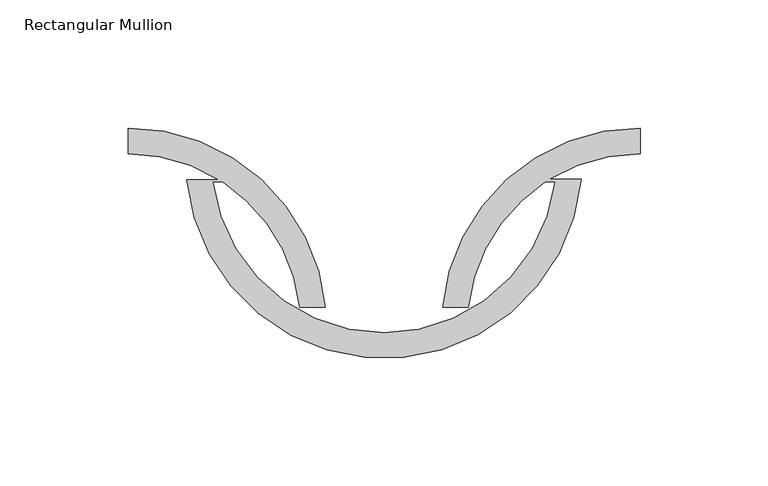
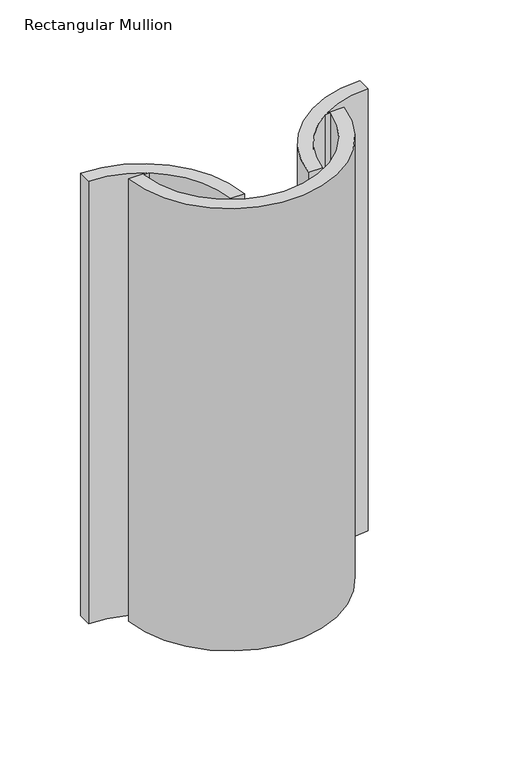
"""IFC4 building model written with IfcOpenShell, lengths in millimetres: member geometry, Rectangular Mullion : Telha Cerâmica - Colonial."""

from ifc_helpers import new_model, si_unit, point, frame, frame_2d, origin, place, context, project, spatial, polyline, circle_curve, trimmed, segment, composite_curve, outline, extrude, source, transform, mapped, element, save


def rectangular_mullion_1220598e(model_context):
    return source(origin(), model_context, "Body", "SweptSolid", [
        extrude(outline(composite_curve([segment(polyline([(-77.1836628, -20.1172602), (-64.5135712, -20.1172602)]), True, "CONTINUOUS"), segment(trimmed(circle_curve(frame_2d((-100.058911, -77.5)), 67.5), [point((-64.5135712, -20.1172602))], [point((-100.058911, -10.0))], True, "CARTESIAN"), True, "CONTINUOUS"), segment(polyline([(-100.058911, -10.0), (-100.058911, 0.0)]), True, "CONTINUOUS"), segment(trimmed(circle_curve(frame_2d((-100.058911, -77.5)), 77.5), [point((-100.058911, 0.0))], [point((-22.9226679, -70.0))], False, "CARTESIAN"), True, "CONTINUOUS"), segment(polyline([(-22.9226679, -70.0), (-32.9768716, -70.0)]), True, "CONTINUOUS"), segment(trimmed(circle_curve(frame_2d((-100.058911, -77.5)), 67.5), [point((-32.9768716, -70.0))], [point((-63.1265403, -21.0))], True, "CARTESIAN"), True, "CONTINUOUS"), segment(polyline([(-63.1265403, -21.0), (-67.0215871, -21.0)]), True, "CONTINUOUS"), segment(trimmed(circle_curve(frame_2d((-0.058911, -12.5)), 67.5), [point((-67.0215871, -21.0))], [point((66.9037652, -21.0))], True, "CARTESIAN"), True, "CONTINUOUS"), segment(polyline([(66.9037652, -21.0), (63.0087184, -21.0)]), True, "CONTINUOUS"), segment(trimmed(circle_curve(frame_2d((99.941089, -77.5)), 67.5), [point((63.0087184, -21.0))], [point((32.8590497, -70.0))], True, "CARTESIAN"), True, "CONTINUOUS"), segment(polyline([(32.8590497, -70.0), (22.8048459, -70.0)]), True, "CONTINUOUS"), segment(trimmed(circle_curve(frame_2d((99.941089, -77.5)), 77.5), [point((22.8048459, -70.0))], [point((99.941089, 0.0))], False, "CARTESIAN"), True, "CONTINUOUS"), segment(polyline([(99.941089, 0.0), (99.941089, -10.0)]), True, "CONTINUOUS"), segment(trimmed(circle_curve(frame_2d((99.941089, -77.5)), 67.5), [point((99.941089, -10.0))], [point((64.58575, -20.0))], True, "CARTESIAN"), True, "CONTINUOUS"), segment(polyline([(64.58575, -20.0), (77.0773321, -20.0)]), True, "CONTINUOUS"), segment(trimmed(circle_curve(frame_2d((-0.058911, -12.5)), 77.5), [point((77.0773321, -20.0))], [point((-77.1836628, -20.1172602))], False, "CARTESIAN"), True, "CONTINUOUS")], self_intersect=False)), frame((0.0, 0.0, -334.7005384), z_axis=(0.0, 0.0, 1.0), x_axis=(1.0, 0.0, 0.0)), (0.0, 0.0, 1.0), 334.7005384),
    ])


if __name__ == "__main__":
    model = new_model("IFC4")
    model_context = context("Model", 3, world=origin())
    ifc_project = project(units=[si_unit("LENGTHUNIT", "METRE", prefix="MILLI")], contexts=[model_context])
    site = spatial("IfcSite", under=ifc_project)
    building = spatial("IfcBuilding", under=site)
    placement = place(None, origin())
    rectangular_mullion_shape = rectangular_mullion_1220598e(model_context)
    element("IfcMember", 1, ObjectType="Rectangular Mullion : Telha Cerâmica - Colonial", at=placement, inside=building, context=model_context, shape_type="MappedRepresentation", body=[
        mapped(rectangular_mullion_shape, transform((0.0, 0.0, 0.0), x_axis=(1.0, 0.0, 0.0), y_axis=(0.0, 1.0, 0.0), z_axis=(0.0, 0.0, 1.0))),
    ])
    save(model, "model.ifc")

# Revit data of these elements
# Type "Rectangular Mullion : Telha Cerâmica - Colonial"
#   built-in parameter 1007322 = 0.0328084 (stored number, unit not read)
#   built-in parameter 1007321 = 0.327891 (stored number, unit not read)
#   built-in parameter 1007320 = 0.328277 (stored number, unit not read)
# Element 1 (IfcMember, "Rectangular Mullion : Telha Cerâmica - Colonial")
#   Materials on its faces: "Telha - Cerâmica"
# Materials
#   "Telha - Cerâmica": class "Cerâmica", colour RGB 68 35 31, transparency 0, Description = "Interior finish", Cost = 0
